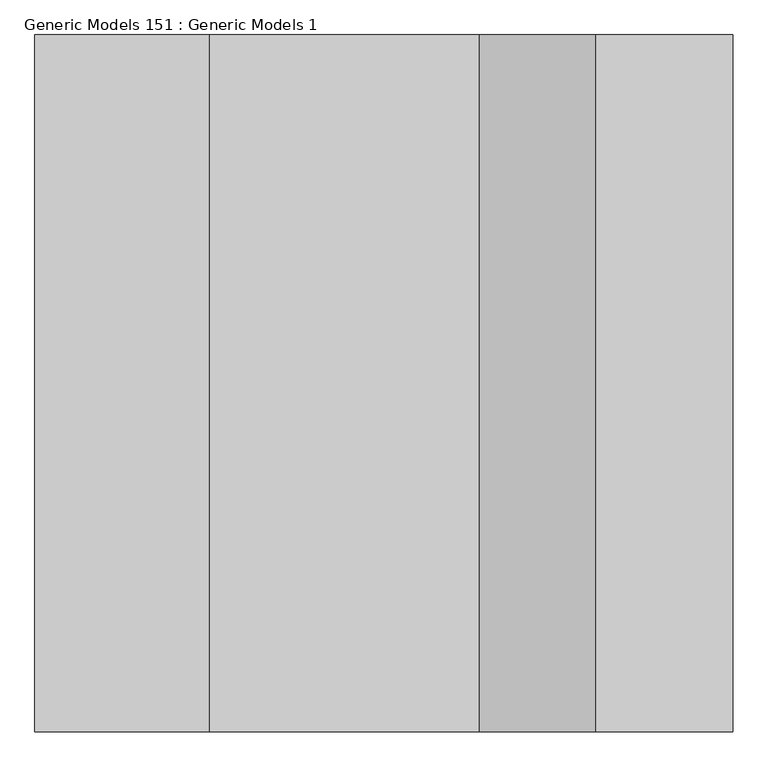
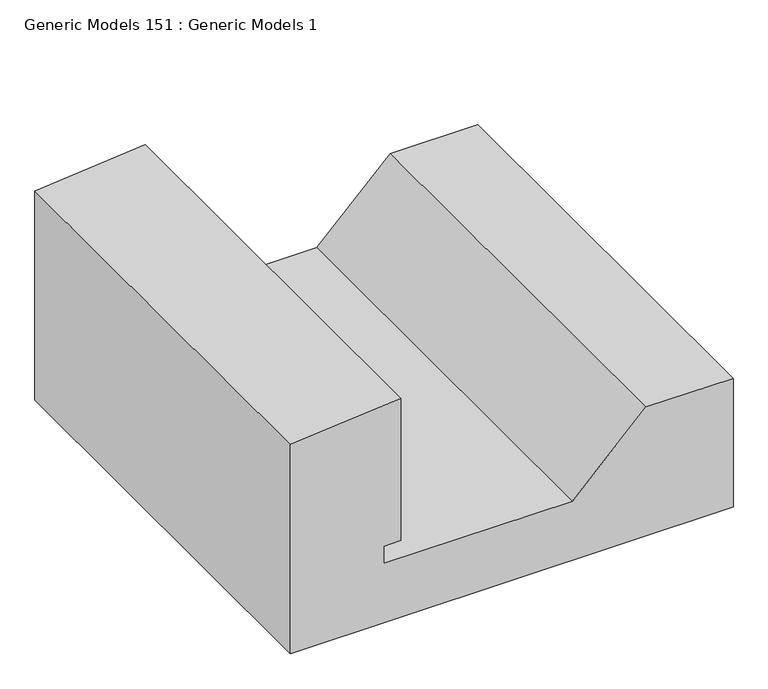
"""IFC4 building model written with IfcOpenShell, lengths in millimetres: proxy geometry, Generic Models 151 : Generic Models 1."""

import ifcopenshell
import ifcopenshell.guid

model = None  # the IFC model being written
_history = None  # IfcOwnerHistory: only IFC2X3 demands one
_inside = {}  # id of a spatial element -> (the spatial element, [elements in it])
_under = {}  # id of a project, library or spatial element -> (it, [spatial elements below it])
_declared = {}  # id of a project -> (the project, [libraries it declares])
_typed = {}  # id of a type object -> (the type object, [elements of that type])
_made_of = {}  # id of a material, layer set ... -> (it, [elements and type objects made of it])


def new_model(schema):
    """Start an empty IFC model of exactly this schema.

    Asked for "IFC4X3", IfcOpenShell would pick the latest addendum, in which some entities
    have other attributes; the version numbers below select the first issue.
    IFC2X3 requires an IfcOwnerHistory on every rooted entity: one is made here for all.
    """
    global model, _history
    if schema == "IFC4X3":
        model = ifcopenshell.file(schema_version=(4, 3, 0, 0))
    else:
        model = ifcopenshell.file(schema=schema)
    _inside.clear()
    _under.clear()
    _declared.clear()
    _typed.clear()
    _made_of.clear()
    _history = None
    if model.schema == "IFC2X3":
        org = make("IfcOrganization", Name="unknown")
        user = make(
            "IfcPersonAndOrganization",
            ThePerson=make("IfcPerson", FamilyName="unknown"),
            TheOrganization=org,
        )
        app = make(
            "IfcApplication",
            ApplicationDeveloper=org,
            Version="unknown",
            ApplicationFullName="unknown",
            ApplicationIdentifier="unknown",
        )
        _history = make(
            "IfcOwnerHistory",
            OwningUser=user,
            OwningApplication=app,
            ChangeAction="ADDED",
            CreationDate=0,
        )
    return model


def make(cls, **values):
    """One entity of the class cls with the attributes given. An attribute that is None is left unset."""
    return model.create_entity(
        cls, **{name: value for name, value in values.items() if value is not None}
    )


def rooted(cls, **values):
    """An entity with a GlobalId (a new one), such as an element, a storey or a relation."""
    return make(cls, GlobalId=ifcopenshell.guid.new(), OwnerHistory=_history, **values)


def si_unit(unit_type, name, prefix=None):
    """IfcSIUnit, for example si_unit("LENGTHUNIT", "METRE", prefix="MILLI")."""
    return make("IfcSIUnit", UnitType=unit_type, Prefix=prefix, Name=name)


def assignment(units):
    """IfcUnitAssignment: the units of a project."""
    return None if units is None else make("IfcUnitAssignment", Units=units)


def point(xyz):
    """IfcCartesianPoint."""
    return None if xyz is None else make("IfcCartesianPoint", Coordinates=xyz)


def direction(xyz):
    """IfcDirection."""
    return None if xyz is None else make("IfcDirection", DirectionRatios=xyz)


def frame(location, z_axis=None, x_axis=None):
    """IfcAxis2Placement3D, a coordinate frame: its origin and axes. An axis left out is left unset."""
    return make(
        "IfcAxis2Placement3D",
        Location=point(location),
        Axis=direction(z_axis),
        RefDirection=direction(x_axis),
    )


def origin():
    """The frame at (0, 0, 0) with its axes left unset."""
    return frame((0.0, 0.0, 0.0))


def place(relative_to, where):
    """IfcLocalPlacement: puts the frame where relative to a parent placement (None: the world)."""
    return make(
        "IfcLocalPlacement", PlacementRelTo=relative_to, RelativePlacement=where
    )


def context(
    kind, dimensions, precision=None, world=None, true_north=None, identifier=None
):
    """IfcGeometricRepresentationContext, for example the 3D "Model" context."""
    return make(
        "IfcGeometricRepresentationContext",
        ContextIdentifier=identifier,
        ContextType=kind,
        CoordinateSpaceDimension=dimensions,
        Precision=precision,
        WorldCoordinateSystem=world,
        TrueNorth=true_north,
    )


def project(units=None, contexts=None):
    """IfcProject with its units and contexts."""
    return rooted(
        "IfcProject",
        Name="project",
        RepresentationContexts=contexts,
        UnitsInContext=assignment(units),
    )


def spatial(cls, under=None, at=None, **own):
    """A site, building, storey or space (cls), placed at a placement, below another one or the project."""
    s = rooted(cls, ObjectPlacement=at, **own)
    if under is not None:
        _under.setdefault(under.id(), (under, []))[1].append(s)
    return s


def polyline(points):
    """IfcPolyline through the points."""
    return make("IfcPolyline", Points=[point(p) for p in points])


def outline(outer, holes=None, kind="AREA"):
    """IfcArbitraryClosedProfileDef: a profile drawn as a closed curve; with holes, ...WithVoids."""
    if holes is None:
        return make("IfcArbitraryClosedProfileDef", ProfileType=kind, OuterCurve=outer)
    return make(
        "IfcArbitraryProfileDefWithVoids",
        ProfileType=kind,
        OuterCurve=outer,
        InnerCurves=holes,
    )


def extrude(swept, where, along, depth):
    """IfcExtrudedAreaSolid: the profile swept, set in the frame where, extruded along a direction by depth."""
    return make(
        "IfcExtrudedAreaSolid",
        SweptArea=swept,
        Position=where,
        ExtrudedDirection=direction(along),
        Depth=depth,
    )


def shape(context_of_items, identifier, shape_type, items):
    """IfcShapeRepresentation: the items that make up one representation, for example the "Body"."""
    return make(
        "IfcShapeRepresentation",
        ContextOfItems=context_of_items,
        RepresentationIdentifier=identifier,
        RepresentationType=shape_type,
        Items=items,
    )


def source(mapping_origin, context_of_items, identifier, shape_type, items):
    """IfcRepresentationMap: a shape defined once, which mapped items show again and again."""
    return make(
        "IfcRepresentationMap",
        MappingOrigin=mapping_origin,
        MappedRepresentation=shape(context_of_items, identifier, shape_type, items),
    )


def transform(
    local_origin,
    x_axis=None,
    y_axis=None,
    z_axis=None,
    scale=None,
    scale2=None,
    scale3=None,
    uniform=True,
):
    """IfcCartesianTransformationOperator3D, or its non-uniform kind. x_axis, y_axis, z_axis: its Axis1, 2, 3."""
    if uniform:
        return make(
            "IfcCartesianTransformationOperator3D",
            Axis1=direction(x_axis),
            Axis2=direction(y_axis),
            LocalOrigin=point(local_origin),
            Scale=scale,
            Axis3=direction(z_axis),
        )
    return make(
        "IfcCartesianTransformationOperator3DnonUniform",
        Axis1=direction(x_axis),
        Axis2=direction(y_axis),
        LocalOrigin=point(local_origin),
        Scale=scale,
        Axis3=direction(z_axis),
        Scale2=scale2,
        Scale3=scale3,
    )


def mapped(mapping_source, mapping_target):
    """IfcMappedItem: shows the shape of a source again, moved by a transform."""
    return make(
        "IfcMappedItem", MappingSource=mapping_source, MappingTarget=mapping_target
    )


def made_of(thing, what):
    """Note that an element or type object is made of a material, layer set ...; save() writes the relation."""
    if what is not None:
        _made_of.setdefault(what.id(), (what, []))[1].append(thing)
    return thing


def element(
    cls,
    number,
    at=None,
    inside=None,
    cuts=None,
    type_object=None,
    material=None,
    context=None,
    identifier="Body",
    shape_type=None,
    held_by="IfcProductDefinitionShape",
    body=None,
    shapes=None,
    **own,
):
    """One element of the class cls, such as IfcWall. Its Tag is "e" and its number.

    at: its placement. inside: the storey or other place that contains it. cuts: it is an
    opening in that element (IfcRelVoidsElement). A single representation is given by context,
    identifier, shape_type and body (its items); several are given by shapes. held_by: the class
    of the entity that holds the representations. save() writes the other relations.
    """
    e = rooted(cls, Tag="e%d" % number, ObjectPlacement=at, **own)
    if body is not None:
        shapes = [shape(context, identifier, shape_type, body)]
    if shapes is not None:
        e.Representation = make(held_by, Representations=shapes)
    if inside is not None:
        _inside.setdefault(inside.id(), (inside, []))[1].append(e)
    if cuts is not None:
        rooted(
            "IfcRelVoidsElement", RelatingBuildingElement=cuts, RelatedOpeningElement=e
        )
    if type_object is not None:
        _typed.setdefault(type_object.id(), (type_object, []))[1].append(e)
    return made_of(e, material)


def aggregate(whole, parts):
    """IfcRelAggregates: a whole, such as a stair, and the parts it consists of."""
    return rooted("IfcRelAggregates", RelatingObject=whole, RelatedObjects=parts)


def save(model, path):
    """Write the relations noted so far, then the file.

    IfcRelAggregates (storeys below a building ...), IfcRelContainedInSpatialStructure (elements
    in a storey), IfcRelDefinesByType, IfcRelAssociatesMaterial and IfcRelDeclares: one each for
    every whole, place, type object, material and project.
    """
    for whole, parts in _under.values():
        aggregate(whole, parts)
    for where, things in _inside.values():
        rooted(
            "IfcRelContainedInSpatialStructure",
            RelatedElements=things,
            RelatingStructure=where,
        )
    for kind, things in _typed.values():
        rooted("IfcRelDefinesByType", RelatedObjects=things, RelatingType=kind)
    for what, things in _made_of.values():
        rooted("IfcRelAssociatesMaterial", RelatedObjects=things, RelatingMaterial=what)
    for by, libraries in _declared.values():
        rooted("IfcRelDeclares", RelatingContext=by, RelatedDefinitions=libraries)
    model.write(path)


def generic_models_151_generic_models_1_08f1ca75(model_context):
    return source(origin(), model_context, "Body", "SweptSolid", [
        extrude(outline(polyline([(-76.2, 51566.7625), (-685.8, 51566.7625), (-685.8, 52787.3395874), (-310.1710164, 52787.3395874), (-310.1710164, 52546.8563593), (-513.3710164, 52343.6563593), (-513.3710164, 51824.8420742), (-462.5710164, 51824.8420742), (-462.5710164, 51871.5625), (-47.9216734, 51871.5625), (-76.2, 51566.7625)])), frame((0.0, 0.0, 0.0), z_axis=(0.0, 1.0, 0.0), x_axis=(0.0, 0.0, 1.0)), (0.0, 0.0, 1.0), 1219.2),
    ])


if __name__ == "__main__":
    model = new_model("IFC4")
    model_context = context("Model", 3, world=origin())
    ifc_project = project(units=[si_unit("LENGTHUNIT", "METRE", prefix="MILLI")], contexts=[model_context])
    site = spatial("IfcSite", under=ifc_project)
    building = spatial("IfcBuilding", under=site)
    placement = place(None, origin())
    generic_models_151_generic_models_1_shape = generic_models_151_generic_models_1_08f1ca75(model_context)
    element("IfcBuildingElementProxy", 1, Name="Generic Models 151 : Generic Models 1", ObjectType="Generic Models 151 : Generic Models 1", at=placement, inside=building, context=model_context, shape_type="MappedRepresentation", body=[
        mapped(generic_models_151_generic_models_1_shape, transform((0.0, 0.0, 0.0), x_axis=(1.0, 0.0, 0.0), y_axis=(0.0, 1.0, 0.0), z_axis=(0.0, 0.0, 1.0))),
    ])
    save(model, "model.ifc")

# Revit data of these elements
# Element 1 (IfcBuildingElementProxy, "Generic Models 151 : Generic Models 1")
#   Materials on its faces: "GRADE (SLOPE 2% MIN AWAY FROM BUILDING)"
# Materials
#   "GRADE (SLOPE 2% MIN AWAY FROM BUILDING)": class "Generic", colour RGB 211 211 211, transparency 0, Description = "Soil", Cost = 0
